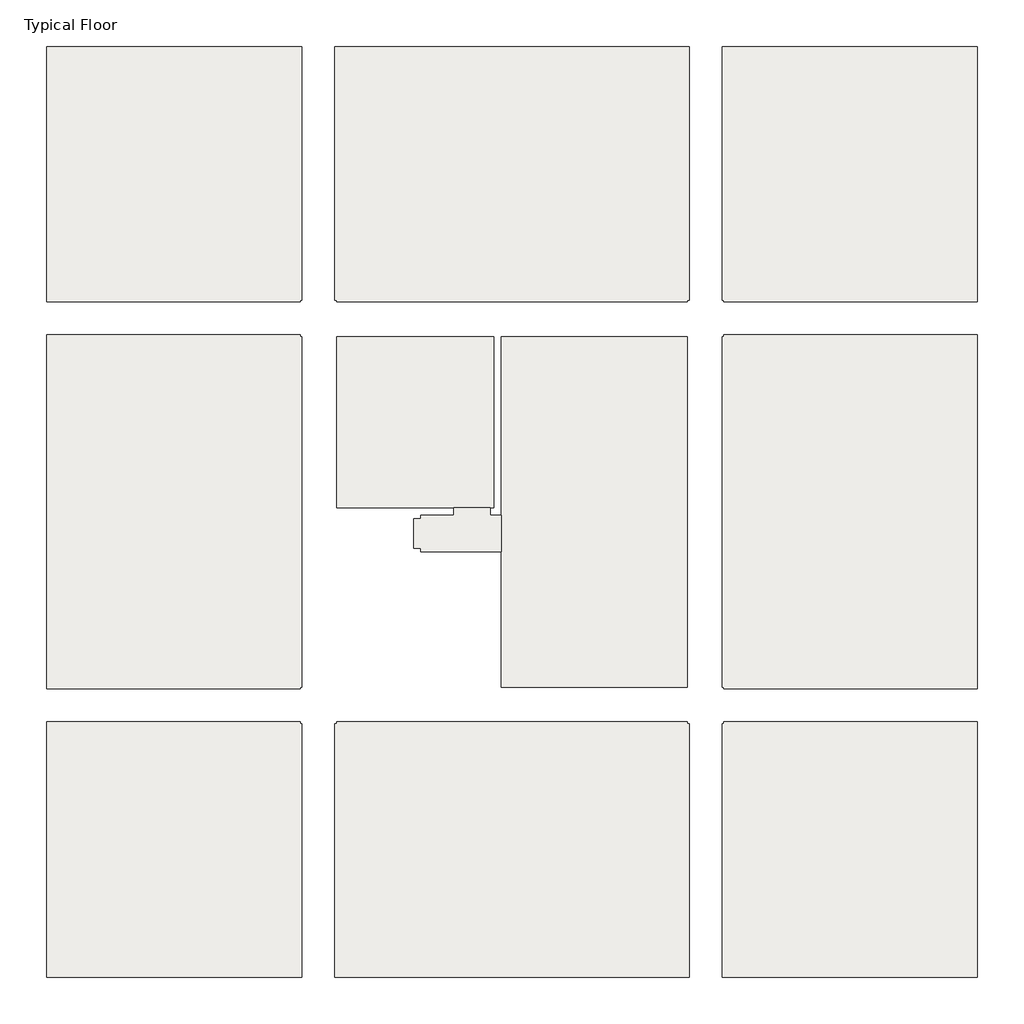
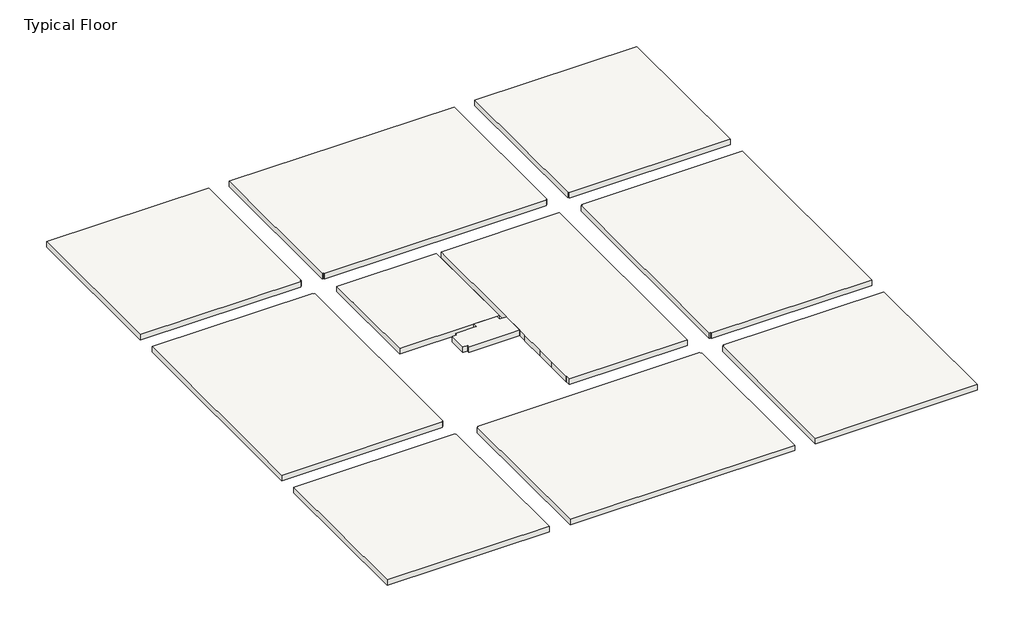
# One storey: 11 slabs.
"""IFC4 building model written with IfcOpenShell, lengths in millimetres."""

from ifc_helpers import new_model, si_unit, frame, origin, place, context, project, spatial, polyline, outline, extrude, faceted_brep, element, save

model = new_model("IFC4")

# Units and contexts
model_context = context("Model", 3, world=origin())
ifc_project = project(units=[si_unit("LENGTHUNIT", "METRE", prefix="MILLI")], contexts=[model_context])

# Site, building, storey
site = spatial("IfcSite", under=ifc_project)
building = spatial("IfcBuilding", under=site)
storey = spatial("IfcBuildingStorey", under=building, Name="Typical Floor", Elevation=3500.0)

# Slabs
placement = place(None, origin())
element("IfcSlab", 1, ObjectType="25", at=placement, inside=storey, context=model_context, shape_type="SweptSolid", body=[
    extrude(outline(polyline([(-16590.3344173, -8548.2491126), (-23590.3344173, -8548.2491126), (-23590.3344173, -1548.2491126), (-16640.3344173, -1548.2491126), (-16640.3344173, -1598.2491126), (-16590.3344173, -1598.2491126), (-16590.3344173, -8548.2491126)])), frame((0.0, 0.0, 3250.0), z_axis=(0.0, 0.0, 1.0), x_axis=(1.0, 0.0, 0.0)), (0.0, 0.0, 1.0), 250.0),
])
element("IfcSlab", 2, ObjectType="25", at=placement, inside=storey, context=model_context, shape_type="SweptSolid", body=[
    extrude(outline(polyline([(-5980.9538985, -8548.2491126), (-15690.3344173, -8548.2491126), (-15690.3344173, -1598.2491126), (-15640.3344173, -1598.2491126), (-15640.3344173, -1548.2491126), (-6030.9538985, -1548.2491126), (-6030.9538985, -1598.2491126), (-5980.9538985, -1598.2491126), (-5980.9538985, -8548.2491126)])), frame((0.0, 0.0, 3250.0), z_axis=(0.0, 0.0, 1.0), x_axis=(1.0, 0.0, 0.0)), (0.0, 0.0, 1.0), 250.0),
])
element("IfcSlab", 3, ObjectType="25", at=placement, inside=storey, context=model_context, shape_type="SweptSolid", body=[
    extrude(outline(polyline([(-5030.9538985, -1598.2491126), (-5030.9538985, -1548.2491126), (1919.0461015, -1548.2491126), (1919.0461015, -8548.2491126), (-5080.9538985, -8548.2491126), (-5080.9538985, -1598.2491126), (-5030.9538985, -1598.2491126)])), frame((0.0, 0.0, 3250.0), z_axis=(0.0, 0.0, 1.0), x_axis=(1.0, 0.0, 0.0)), (0.0, 0.0, 1.0), 250.0),
])
element("IfcSlab", 4, ObjectType="25", at=placement, inside=storey, context=model_context, shape_type="SweptSolid", body=[
    extrude(outline(polyline([(-5030.9538985, 9003.1817285), (-5030.9538985, 9053.1817285), (1919.0461015, 9053.1817285), (1919.0461015, -648.2491126), (-5030.9538985, -648.2491126), (-5030.9538985, -598.2491126), (-5080.9538985, -598.2491126), (-5080.9538985, 9003.1817285), (-5030.9538985, 9003.1817285)])), frame((0.0, 0.0, 3250.0), z_axis=(0.0, 0.0, 1.0), x_axis=(1.0, 0.0, 0.0)), (0.0, 0.0, 1.0), 250.0),
])
element("IfcSlab", 5, ObjectType="25", at=placement, inside=storey, context=model_context, shape_type="SweptSolid", body=[
    extrude(outline(polyline([(-5030.9538985, 10003.1817285), (-5080.9538985, 10003.1817285), (-5080.9538985, 16952.588413), (1919.0461015, 16952.588413), (1919.0461015, 9953.1817285), (-5030.9538985, 9953.1817285), (-5030.9538985, 10003.1817285)])), frame((0.0, 0.0, 3250.0), z_axis=(0.0, 0.0, 1.0), x_axis=(1.0, 0.0, 0.0)), (0.0, 0.0, 1.0), 250.0),
])
element("IfcSlab", 6, ObjectType="25", at=placement, inside=storey, context=model_context, shape_type="SweptSolid", body=[
    extrude(outline(polyline([(-15640.3344173, 10003.1817285), (-15690.3344173, 10003.1817285), (-15690.3344173, 16952.588413), (-5980.9538985, 16952.588413), (-5980.9538985, 10003.1817285), (-6030.9538985, 10003.1817285), (-6030.9538985, 9953.1817285), (-15640.3344173, 9953.1817285), (-15640.3344173, 10003.1817285)])), frame((0.0, 0.0, 3250.0), z_axis=(0.0, 0.0, 1.0), x_axis=(1.0, 0.0, 0.0)), (0.0, 0.0, 1.0), 250.0),
])
element("IfcSlab", 7, ObjectType="25", at=placement, inside=storey, context=model_context, shape_type="SweptSolid", body=[
    extrude(outline(polyline([(-23590.3344173, 16953.1817285), (-16590.3344173, 16953.1817285), (-16590.3344173, 10003.1817285), (-16640.3344173, 10003.1817285), (-16640.3344173, 9953.1817285), (-23590.3344173, 9953.1817285), (-23590.3344173, 16953.1817285)])), frame((0.0, 0.0, 3250.0), z_axis=(0.0, 0.0, 1.0), x_axis=(1.0, 0.0, 0.0)), (0.0, 0.0, 1.0), 250.0),
])
element("IfcSlab", 8, ObjectType="25", at=placement, inside=storey, context=model_context, shape_type="SweptSolid", body=[
    extrude(outline(polyline([(-16640.3344173, 9053.1817285), (-16640.3344173, 9003.1817285), (-16590.3344173, 9003.1817285), (-16590.3344173, -598.2491126), (-16640.3344173, -598.2491126), (-16640.3344173, -648.2491126), (-23590.3344173, -648.2491126), (-23590.3344173, 9053.1817285), (-16640.3344173, 9053.1817285)])), frame((0.0, 0.0, 3250.0), z_axis=(0.0, 0.0, 1.0), x_axis=(1.0, 0.0, 0.0)), (0.0, 0.0, 1.0), 250.0),
])
element("IfcSlab", 9, ObjectType="25", at=placement, inside=storey, context=model_context, shape_type="Brep", body=[
    faceted_brep([(-11331.5944827, 9003.1817285, 3250.0), (-11331.5944827, 4310.3323713, 3250.0), (-11432.1347032, 4310.3323713, 3250.0), (-12431.1134644, 4310.3323713, 3250.0), (-15631.2318689, 4310.3323713, 3250.0), (-15631.2318689, 9003.1817285, 3250.0), (-11331.5944827, 9003.1817285, 3500.0), (-15631.2318689, 9003.1817285, 3500.0), (-15631.2318689, 4310.3323713, 3500.0), (-12431.1134644, 4310.3323713, 3500.0), (-11432.1347032, 4310.3323713, 3500.0), (-11331.5944827, 4310.3323713, 3500.0)], [[[0, 1, 2, 3, 4, 5]], [[6, 7, 8, 9, 10, 11]], [[1, 0, 6, 11]], [[4, 3, 2, 1, 11, 10, 9, 8]], [[5, 4, 8, 7]], [[0, 5, 7, 6]]]),
])
element("IfcSlab", 10, ObjectType="25", at=placement, inside=storey, context=model_context, shape_type="Brep", body=[
    faceted_brep([(-6030.9538985, 9003.1817285, 3250.0), (-6030.9538985, -598.2491126, 3250.0), (-11131.5666819, -598.2491126, 3250.0), (-11131.5666819, -391.4214954, 3250.0), (-11136.5944827, -391.4214954, 3250.0), (-11136.5944827, 709.1483263, 3250.0), (-11132.6601232, 709.1483263, 3250.0), (-11132.6601232, 1608.6525075, 3250.0), (-11136.5944827, 1608.6525075, 3250.0), (-11136.5944827, 2709.2371297, 3250.0), (-11130.6176456, 2709.2371297, 3250.0), (-11130.6176456, 3109.2371297, 3250.0), (-11136.5944827, 3109.2371297, 3250.0), (-11136.5944827, 4110.3323713, 3250.0), (-11131.5944827, 4110.3323713, 3250.0), (-11131.5944827, 9003.1817285, 3250.0), (-6030.9538985, -598.2491126, 3500.0), (-6030.9538985, 9003.1817285, 3500.0), (-11131.5944827, 9003.1817285, 3500.0), (-11131.5944827, 4310.3323713, 3500.0), (-11131.5944827, 4110.3323713, 3500.0), (-11136.5944827, 4110.3323713, 3500.0), (-11136.5944827, 3109.2371297, 3500.0), (-11130.6176456, 3109.2371297, 3500.0), (-11130.6176456, 2709.2371297, 3500.0), (-11136.5944827, 2709.2371297, 3500.0), (-11136.5944827, 1608.6525075, 3500.0), (-11132.6601232, 1608.6525075, 3500.0), (-11132.6601232, 709.1483263, 3500.0), (-11136.5944827, 709.1483263, 3500.0), (-11136.5944827, -391.4214954, 3500.0), (-11131.5666819, -391.4214954, 3500.0), (-11131.5666819, -598.2491126, 3500.0)], [[[0, 1, 2, 3, 4, 5, 6, 7, 8, 9, 10, 11, 12, 13, 14, 15]], [[16, 17, 18, 19, 20, 21, 22, 23, 24, 25, 26, 27, 28, 29, 30, 31, 32]], [[1, 0, 17, 16]], [[1, 16, 32, 2]], [[25, 9, 8, 26]], [[12, 22, 21, 13]], [[4, 30, 29, 5]], [[17, 0, 15, 18]], [[18, 15, 14, 20, 19]], [[10, 24, 23, 11]], [[24, 10, 9, 25]], [[11, 23, 22, 12]], [[31, 3, 2, 32]], [[3, 31, 30, 4]], [[20, 14, 13, 21]], [[6, 28, 27, 7]], [[7, 27, 26, 8]], [[28, 6, 5, 29]]]),
])
element("IfcSlab", 11, ObjectType="25", at=placement, inside=storey, context=model_context, shape_type="Brep", body=[
    faceted_brep([(-13530.6176456, 3208.7117097, 3250.0), (-13530.6176456, 4008.7413108, 3250.0), (-13330.6176456, 4008.7413108, 3250.0), (-13330.6176456, 4110.3323713, 3250.0), (-12431.1134644, 4110.3323713, 3250.0), (-12431.1134644, 4310.3323713, 3250.0), (-11432.1347032, 4310.3323713, 3250.0), (-11432.1347032, 4110.3323713, 3250.0), (-11136.5944827, 4110.3323713, 3250.0), (-11136.5944827, 3109.2371297, 3250.0), (-13330.6176456, 3109.2371297, 3250.0), (-13330.6176456, 3208.7117097, 3250.0), (-13530.6176456, 4008.7413108, 3500.0), (-13530.6176456, 3208.7117097, 3500.0), (-13330.6176456, 3208.7117097, 3500.0), (-13330.6176456, 3109.2371297, 3500.0), (-11330.6176456, 3109.2371297, 3500.0), (-11136.5944827, 3109.2371297, 3500.0), (-11136.5944827, 4110.3323713, 3500.0), (-11432.1347032, 4110.3323713, 3500.0), (-11432.1347032, 4310.3323713, 3500.0), (-12431.1134644, 4310.3323713, 3500.0), (-12431.1134644, 4110.3323713, 3500.0), (-13330.6176456, 4110.3323713, 3500.0), (-13330.6176456, 4008.7413108, 3500.0)], [[[0, 1, 2, 3, 4, 5, 6, 7, 8, 9, 10, 11]], [[12, 13, 14, 15, 16, 17, 18, 19, 20, 21, 22, 23, 24]], [[1, 0, 13, 12]], [[2, 1, 12, 24]], [[3, 2, 24, 23]], [[4, 3, 23, 22]], [[5, 4, 22, 21]], [[5, 21, 20, 6]], [[7, 19, 18, 8]], [[15, 10, 9, 17, 16]], [[11, 10, 15, 14]], [[0, 11, 14, 13]], [[19, 7, 6, 20]], [[9, 8, 18, 17]]]),
])

save(model, "model.ifc")

# Revit data of these elements
# Type "25"
#   Function = 0
#   Layers, outside or top first: 25 cm "Concrete" (function 1)
# Element 1 (IfcSlab, "25")
#   Mark = "S1"
#   SOFiSTiK_AMG_Comments = ""
#   Height Offset From Level = 0 cm
#   built-in parameter 1001954 = 1
#   SOFiSTiK_AMG_Scheduled = yes
#   SOFiSTiK_AMG_Adjusted = yes
#   Phase Created = New Construction
#   Materials on its faces: "Concrete"
# Element 2 (IfcSlab, "25")
#   Mark = "S2"
#   SOFiSTiK_AMG_Comments = ""
#   Height Offset From Level = 0 cm
#   built-in parameter 1001954 = 1
#   SOFiSTiK_AMG_Scheduled = yes
#   SOFiSTiK_AMG_Adjusted = yes
#   Phase Created = New Construction
#   Materials on its faces: "Concrete"
# Element 3 (IfcSlab, "25")
#   Mark = "S3"
#   SOFiSTiK_AMG_Comments = ""
#   Height Offset From Level = 0 cm
#   built-in parameter 1001954 = 1
#   SOFiSTiK_AMG_Scheduled = yes
#   SOFiSTiK_AMG_Adjusted = yes
#   Phase Created = New Construction
#   Materials on its faces: "Concrete"
# Element 4 (IfcSlab, "25")
#   Mark = "S4"
#   SOFiSTiK_AMG_Comments = ""
#   Height Offset From Level = 0 cm
#   built-in parameter 1001954 = 1
#   SOFiSTiK_AMG_Scheduled = yes
#   SOFiSTiK_AMG_Adjusted = yes
#   Phase Created = New Construction
#   Materials on its faces: "Concrete"
# Element 5 (IfcSlab, "25")
#   Mark = "S5"
#   SOFiSTiK_AMG_Comments = ""
#   built-in parameter 1001955 = 1.5708 (stored number, unit not read)
#   Height Offset From Level = 0 cm
#   built-in parameter 1001954 = 1
#   SOFiSTiK_AMG_Scheduled = yes
#   SOFiSTiK_AMG_Adjusted = yes
#   Phase Created = New Construction
#   Materials on its faces: "Concrete"
# Element 6 (IfcSlab, "25")
#   Mark = "S6"
#   SOFiSTiK_AMG_Comments = ""
#   built-in parameter 1001955 = 1.5708 (stored number, unit not read)
#   Height Offset From Level = 0 cm
#   built-in parameter 1001954 = 1
#   SOFiSTiK_AMG_Scheduled = yes
#   SOFiSTiK_AMG_Adjusted = yes
#   Phase Created = New Construction
#   Materials on its faces: "Concrete"
# Element 7 (IfcSlab, "25")
#   Mark = "S7"
#   SOFiSTiK_AMG_Comments = ""
#   built-in parameter 1001955 = 3.14159 (stored number, unit not read)
#   Height Offset From Level = 0 cm
#   built-in parameter 1001954 = 1
#   SOFiSTiK_AMG_Scheduled = yes
#   SOFiSTiK_AMG_Adjusted = yes
#   Phase Created = New Construction
#   Materials on its faces: "Concrete"
# Element 8 (IfcSlab, "25")
#   Mark = "S8"
#   SOFiSTiK_AMG_Comments = ""
#   Height Offset From Level = 0 cm
#   built-in parameter 1001954 = 1
#   SOFiSTiK_AMG_Scheduled = yes
#   SOFiSTiK_AMG_Adjusted = yes
#   Phase Created = New Construction
#   Materials on its faces: "Concrete"
# Element 9 (IfcSlab, "25")
#   Mark = "S9"
#   SOFiSTiK_AMG_Comments = ""
#   Height Offset From Level = 0 cm
#   built-in parameter 1001954 = 1
#   SOFiSTiK_AMG_Scheduled = yes
#   SOFiSTiK_AMG_Adjusted = yes
#   Phase Created = New Construction
#   Materials on its faces: "Concrete"
# Element 10 (IfcSlab, "25")
#   Mark = "S10"
#   SOFiSTiK_AMG_Comments = ""
#   Height Offset From Level = 0 cm
#   built-in parameter 1001954 = 1
#   SOFiSTiK_AMG_Scheduled = yes
#   SOFiSTiK_AMG_Adjusted = yes
#   Phase Created = New Construction
#   Materials on its faces: "Concrete"
# Element 11 (IfcSlab, "25")
#   Mark = "S11"
#   SOFiSTiK_AMG_Comments = ""
#   built-in parameter 1001955 = -1.5708 (stored number, unit not read)
#   Height Offset From Level = 0 cm
#   built-in parameter 1001954 = 1
#   SOFiSTiK_AMG_Scheduled = yes
#   SOFiSTiK_AMG_Adjusted = yes
#   Phase Created = New Construction
#   Materials on its faces: "Concrete"
# Materials
#   "Concrete": class "Concrete", colour RGB 192 192 192, transparency 0, Keynote = "01000", Description = "Cast-in-place concrete", Cost = 0
